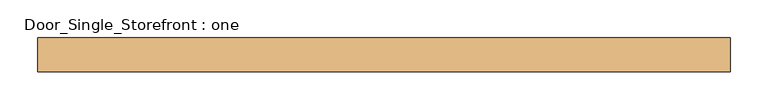
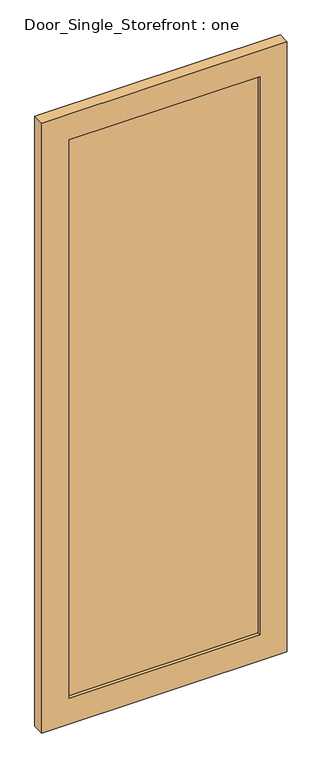
"""IFC4 building model written with IfcOpenShell, lengths in millimetres: door geometry, Door_Single_Storefront : one."""

from ifc_helpers import new_model, si_unit, frame, origin, place, context, project, spatial, polyline, outline, extrude, source, transform, mapped, element, save


def door_single_storefront_one_a54de97d(model_context):
    return source(origin(), model_context, "Body", "SweptSolid", [
        extrude(outline(polyline([(355.6, -6.35), (-355.6, -6.35), (-355.6, 12.7), (355.6, 12.7), (355.6, -6.35)])), frame((0.0, 0.0, 101.6), z_axis=(0.0, 0.0, 1.0), x_axis=(1.0, 0.0, 0.0)), (0.0, 0.0, 1.0), 2197.1),
        extrude(outline(polyline([(2400.3, -457.2), (0.0, -457.2), (0.0, 457.2), (2400.3, 457.2), (2400.3, -457.2)]), holes=[polyline([(101.6, 355.6), (101.6, -355.6), (2298.7, -355.6), (2298.7, 355.6), (101.6, 355.6)])]), frame((0.0, -19.05, 0.0), z_axis=(0.0, 1.0, 0.0), x_axis=(0.0, 0.0, 1.0)), (0.0, 0.0, 1.0), 44.45),
    ])


if __name__ == "__main__":
    model = new_model("IFC4")
    model_context = context("Model", 3, world=origin())
    ifc_project = project(units=[si_unit("LENGTHUNIT", "METRE", prefix="MILLI")], contexts=[model_context])
    site = spatial("IfcSite", under=ifc_project)
    building = spatial("IfcBuilding", under=site)
    placement = place(None, origin())
    door_single_storefront_one_shape = door_single_storefront_one_a54de97d(model_context)
    element("IfcDoor", 1, ObjectType="Door_Single_Storefront : one", at=placement, inside=building, context=model_context, shape_type="MappedRepresentation", body=[
        mapped(door_single_storefront_one_shape, transform((0.0, 0.0, 0.0), x_axis=(1.0, 0.0, 0.0), y_axis=(0.0, 1.0, 0.0), z_axis=(0.0, 0.0, 1.0))),
    ])
    save(model, "model.ifc")

# Revit data of these elements
# Type "Door_Single_Storefront : one"
#   Type Mark = "27"
#   Analytic Construction = "<None>"
#   Stile_Width = 0' - 4"
#   Door_Thickness = 0' - 1 3/4"
#   Door_Offset = 0' - 1"
#   Glass_Material = Glass
#   Frame_Material = Aluminum
#   Function = (empty or 0)
# Element 1 (IfcDoor, "Door_Single_Storefront : one")
#   Materials on its faces: "Aluminum", "Glass"
# Materials
#   "Glass": class "Glass", colour RGB 142 168 196, transparency 0.75, Description = "Soda Lime Glass", Cost = 0
#   "Aluminum": class "Metal", colour RGB 226 226 226, transparency 0, Description = "Aluminum 6061", Cost = 0
